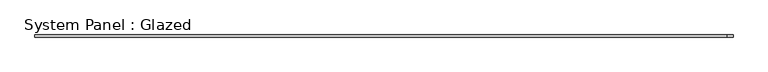
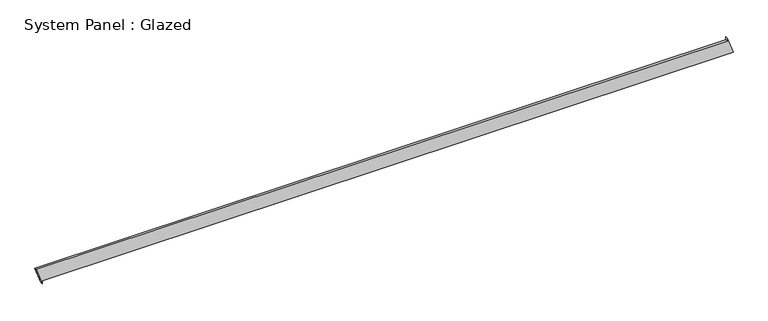
"""IFC4 building model written with IfcOpenShell, lengths in millimetres: plate geometry, System Panel : Glazed."""

import ifcopenshell
import ifcopenshell.guid

model = None  # the IFC model being written
_history = None  # IfcOwnerHistory: only IFC2X3 demands one
_inside = {}  # id of a spatial element -> (the spatial element, [elements in it])
_under = {}  # id of a project, library or spatial element -> (it, [spatial elements below it])
_declared = {}  # id of a project -> (the project, [libraries it declares])
_typed = {}  # id of a type object -> (the type object, [elements of that type])
_made_of = {}  # id of a material, layer set ... -> (it, [elements and type objects made of it])


def new_model(schema):
    """Start an empty IFC model of exactly this schema.

    Asked for "IFC4X3", IfcOpenShell would pick the latest addendum, in which some entities
    have other attributes; the version numbers below select the first issue.
    IFC2X3 requires an IfcOwnerHistory on every rooted entity: one is made here for all.
    """
    global model, _history
    if schema == "IFC4X3":
        model = ifcopenshell.file(schema_version=(4, 3, 0, 0))
    else:
        model = ifcopenshell.file(schema=schema)
    _inside.clear()
    _under.clear()
    _declared.clear()
    _typed.clear()
    _made_of.clear()
    _history = None
    if model.schema == "IFC2X3":
        org = make("IfcOrganization", Name="unknown")
        user = make(
            "IfcPersonAndOrganization",
            ThePerson=make("IfcPerson", FamilyName="unknown"),
            TheOrganization=org,
        )
        app = make(
            "IfcApplication",
            ApplicationDeveloper=org,
            Version="unknown",
            ApplicationFullName="unknown",
            ApplicationIdentifier="unknown",
        )
        _history = make(
            "IfcOwnerHistory",
            OwningUser=user,
            OwningApplication=app,
            ChangeAction="ADDED",
            CreationDate=0,
        )
    return model


def make(cls, **values):
    """One entity of the class cls with the attributes given. An attribute that is None is left unset."""
    return model.create_entity(
        cls, **{name: value for name, value in values.items() if value is not None}
    )


def rooted(cls, **values):
    """An entity with a GlobalId (a new one), such as an element, a storey or a relation."""
    return make(cls, GlobalId=ifcopenshell.guid.new(), OwnerHistory=_history, **values)


def si_unit(unit_type, name, prefix=None):
    """IfcSIUnit, for example si_unit("LENGTHUNIT", "METRE", prefix="MILLI")."""
    return make("IfcSIUnit", UnitType=unit_type, Prefix=prefix, Name=name)


def assignment(units):
    """IfcUnitAssignment: the units of a project."""
    return None if units is None else make("IfcUnitAssignment", Units=units)


def point(xyz):
    """IfcCartesianPoint."""
    return None if xyz is None else make("IfcCartesianPoint", Coordinates=xyz)


def direction(xyz):
    """IfcDirection."""
    return None if xyz is None else make("IfcDirection", DirectionRatios=xyz)


def frame(location, z_axis=None, x_axis=None):
    """IfcAxis2Placement3D, a coordinate frame: its origin and axes. An axis left out is left unset."""
    return make(
        "IfcAxis2Placement3D",
        Location=point(location),
        Axis=direction(z_axis),
        RefDirection=direction(x_axis),
    )


def origin():
    """The frame at (0, 0, 0) with its axes left unset."""
    return frame((0.0, 0.0, 0.0))


def place(relative_to, where):
    """IfcLocalPlacement: puts the frame where relative to a parent placement (None: the world)."""
    return make(
        "IfcLocalPlacement", PlacementRelTo=relative_to, RelativePlacement=where
    )


def context(
    kind, dimensions, precision=None, world=None, true_north=None, identifier=None
):
    """IfcGeometricRepresentationContext, for example the 3D "Model" context."""
    return make(
        "IfcGeometricRepresentationContext",
        ContextIdentifier=identifier,
        ContextType=kind,
        CoordinateSpaceDimension=dimensions,
        Precision=precision,
        WorldCoordinateSystem=world,
        TrueNorth=true_north,
    )


def project(units=None, contexts=None):
    """IfcProject with its units and contexts."""
    return rooted(
        "IfcProject",
        Name="project",
        RepresentationContexts=contexts,
        UnitsInContext=assignment(units),
    )


def spatial(cls, under=None, at=None, **own):
    """A site, building, storey or space (cls), placed at a placement, below another one or the project."""
    s = rooted(cls, ObjectPlacement=at, **own)
    if under is not None:
        _under.setdefault(under.id(), (under, []))[1].append(s)
    return s


def polyline(points):
    """IfcPolyline through the points."""
    return make("IfcPolyline", Points=[point(p) for p in points])


def outline(outer, holes=None, kind="AREA"):
    """IfcArbitraryClosedProfileDef: a profile drawn as a closed curve; with holes, ...WithVoids."""
    if holes is None:
        return make("IfcArbitraryClosedProfileDef", ProfileType=kind, OuterCurve=outer)
    return make(
        "IfcArbitraryProfileDefWithVoids",
        ProfileType=kind,
        OuterCurve=outer,
        InnerCurves=holes,
    )


def extrude(swept, where, along, depth):
    """IfcExtrudedAreaSolid: the profile swept, set in the frame where, extruded along a direction by depth."""
    return make(
        "IfcExtrudedAreaSolid",
        SweptArea=swept,
        Position=where,
        ExtrudedDirection=direction(along),
        Depth=depth,
    )


def shape(context_of_items, identifier, shape_type, items):
    """IfcShapeRepresentation: the items that make up one representation, for example the "Body"."""
    return make(
        "IfcShapeRepresentation",
        ContextOfItems=context_of_items,
        RepresentationIdentifier=identifier,
        RepresentationType=shape_type,
        Items=items,
    )


def source(mapping_origin, context_of_items, identifier, shape_type, items):
    """IfcRepresentationMap: a shape defined once, which mapped items show again and again."""
    return make(
        "IfcRepresentationMap",
        MappingOrigin=mapping_origin,
        MappedRepresentation=shape(context_of_items, identifier, shape_type, items),
    )


def transform(
    local_origin,
    x_axis=None,
    y_axis=None,
    z_axis=None,
    scale=None,
    scale2=None,
    scale3=None,
    uniform=True,
):
    """IfcCartesianTransformationOperator3D, or its non-uniform kind. x_axis, y_axis, z_axis: its Axis1, 2, 3."""
    if uniform:
        return make(
            "IfcCartesianTransformationOperator3D",
            Axis1=direction(x_axis),
            Axis2=direction(y_axis),
            LocalOrigin=point(local_origin),
            Scale=scale,
            Axis3=direction(z_axis),
        )
    return make(
        "IfcCartesianTransformationOperator3DnonUniform",
        Axis1=direction(x_axis),
        Axis2=direction(y_axis),
        LocalOrigin=point(local_origin),
        Scale=scale,
        Axis3=direction(z_axis),
        Scale2=scale2,
        Scale3=scale3,
    )


def mapped(mapping_source, mapping_target):
    """IfcMappedItem: shows the shape of a source again, moved by a transform."""
    return make(
        "IfcMappedItem", MappingSource=mapping_source, MappingTarget=mapping_target
    )


def made_of(thing, what):
    """Note that an element or type object is made of a material, layer set ...; save() writes the relation."""
    if what is not None:
        _made_of.setdefault(what.id(), (what, []))[1].append(thing)
    return thing


def element(
    cls,
    number,
    at=None,
    inside=None,
    cuts=None,
    type_object=None,
    material=None,
    context=None,
    identifier="Body",
    shape_type=None,
    held_by="IfcProductDefinitionShape",
    body=None,
    shapes=None,
    **own,
):
    """One element of the class cls, such as IfcWall. Its Tag is "e" and its number.

    at: its placement. inside: the storey or other place that contains it. cuts: it is an
    opening in that element (IfcRelVoidsElement). A single representation is given by context,
    identifier, shape_type and body (its items); several are given by shapes. held_by: the class
    of the entity that holds the representations. save() writes the other relations.
    """
    e = rooted(cls, Tag="e%d" % number, ObjectPlacement=at, **own)
    if body is not None:
        shapes = [shape(context, identifier, shape_type, body)]
    if shapes is not None:
        e.Representation = make(held_by, Representations=shapes)
    if inside is not None:
        _inside.setdefault(inside.id(), (inside, []))[1].append(e)
    if cuts is not None:
        rooted(
            "IfcRelVoidsElement", RelatingBuildingElement=cuts, RelatedOpeningElement=e
        )
    if type_object is not None:
        _typed.setdefault(type_object.id(), (type_object, []))[1].append(e)
    return made_of(e, material)


def aggregate(whole, parts):
    """IfcRelAggregates: a whole, such as a stair, and the parts it consists of."""
    return rooted("IfcRelAggregates", RelatingObject=whole, RelatedObjects=parts)


def save(model, path):
    """Write the relations noted so far, then the file.

    IfcRelAggregates (storeys below a building ...), IfcRelContainedInSpatialStructure (elements
    in a storey), IfcRelDefinesByType, IfcRelAssociatesMaterial and IfcRelDeclares: one each for
    every whole, place, type object, material and project.
    """
    for whole, parts in _under.values():
        aggregate(whole, parts)
    for where, things in _inside.values():
        rooted(
            "IfcRelContainedInSpatialStructure",
            RelatedElements=things,
            RelatingStructure=where,
        )
    for kind, things in _typed.values():
        rooted("IfcRelDefinesByType", RelatedObjects=things, RelatingType=kind)
    for what, things in _made_of.values():
        rooted("IfcRelAssociatesMaterial", RelatedObjects=things, RelatingMaterial=what)
    for by, libraries in _declared.values():
        rooted("IfcRelDeclares", RelatingContext=by, RelatedDefinitions=libraries)
    model.write(path)


def system_panel_glazed_1248680a(model_context):
    return source(origin(), model_context, "Body", "SweptSolid", [
        extrude(outline(polyline([(0.0, -3958.7701168), (35.3553391, -3958.7701168), (35.3553391, 4027.9908618), (234.4800551, 3958.6624486), (199.124716, 3958.6622495), (199.1697072, -4027.9908618), (0.0, -3958.7701168)])), frame((0.0, -49.5, 0.0), z_axis=(0.0, 1.0, 0.0), x_axis=(0.0, 0.0, 1.0)), (0.0, 0.0, 1.0), 25.0),
    ])


if __name__ == "__main__":
    model = new_model("IFC4")
    model_context = context("Model", 3, world=origin())
    ifc_project = project(units=[si_unit("LENGTHUNIT", "METRE", prefix="MILLI")], contexts=[model_context])
    site = spatial("IfcSite", under=ifc_project)
    building = spatial("IfcBuilding", under=site)
    placement = place(None, origin())
    system_panel_glazed_shape = system_panel_glazed_1248680a(model_context)
    element("IfcPlate", 1, ObjectType="System Panel : Glazed", at=placement, inside=building, context=model_context, shape_type="MappedRepresentation", body=[
        mapped(system_panel_glazed_shape, transform((0.0, 0.0, 0.0), x_axis=(1.0, 0.0, 0.0), y_axis=(0.0, 1.0, 0.0), z_axis=(0.0, 0.0, 1.0))),
    ])
    save(model, "model.ifc")

# Revit data of these elements
# Element 1 (IfcPlate, "System Panel : Glazed")
#   Materials on its faces: "Glass"
# Materials
#   "Glass": class "Glass", colour RGB 218 227 224, transparency 0.85, Description = "Soda Lime Glass", Cost = 0
